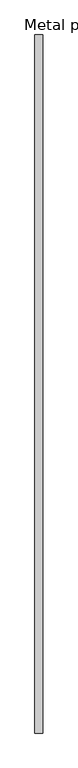
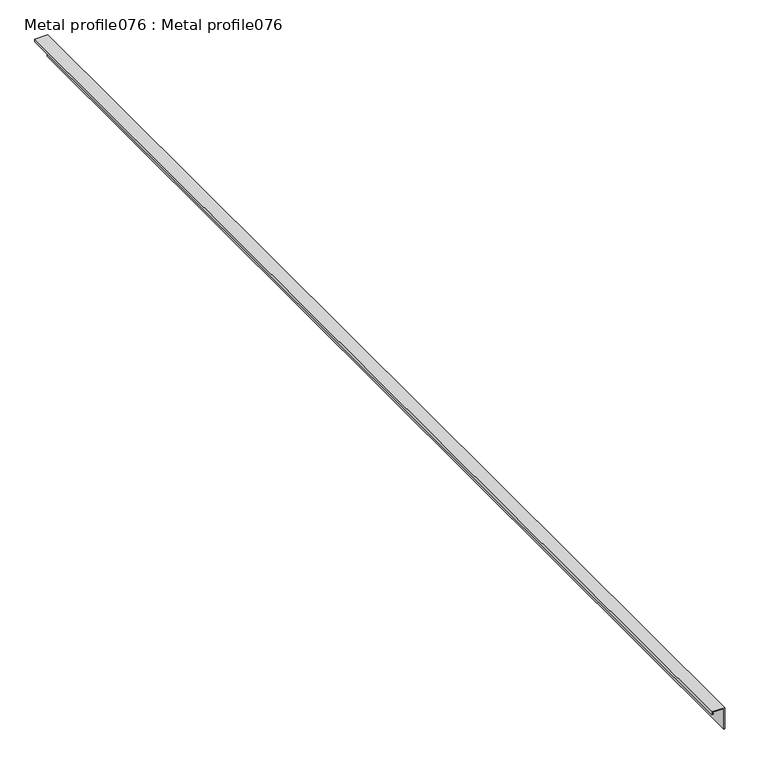
"""IFC4 building model written with IfcOpenShell, lengths in millimetres: proxy geometry, Metal profile076 : Metal profile076."""

from ifc_helpers import new_model, si_unit, frame, origin, place, context, project, spatial, polyline, outline, extrude, source, transform, mapped, element, save


def metal_profile076_metal_profile076_1ce1fb6e(model_context):
    return source(origin(), model_context, "Body", "SweptSolid", [
        extrude(outline(polyline([(40120.4288738, -9897.648077), (40083.5988738, -9897.648077), (40083.5988738, -9896.378077), (40121.6988738, -9896.378077), (40121.6988738, -9918.603077), (40116.9490738, -9918.603077), (40116.9490738, -9915.6006206), (40118.2190738, -9915.6006206), (40118.2190738, -9917.333077), (40120.4288738, -9917.333077), (40120.4288738, -9897.648077)])), frame((0.0, 7182.1531721, 0.0), z_axis=(0.0, 1.0, 0.0), x_axis=(0.0, 0.0, 1.0)), (0.0, 0.0, 1.0), 2000.0),
    ])


if __name__ == "__main__":
    model = new_model("IFC4")
    model_context = context("Model", 3, world=origin())
    ifc_project = project(units=[si_unit("LENGTHUNIT", "METRE", prefix="MILLI")], contexts=[model_context])
    site = spatial("IfcSite", under=ifc_project)
    building = spatial("IfcBuilding", under=site)
    placement = place(None, origin())
    metal_profile076_metal_profile076_shape = metal_profile076_metal_profile076_1ce1fb6e(model_context)
    element("IfcBuildingElementProxy", 1, Name="Metal profile076 : Metal profile076", ObjectType="Metal profile076 : Metal profile076", at=placement, inside=building, context=model_context, shape_type="MappedRepresentation", body=[
        mapped(metal_profile076_metal_profile076_shape, transform((0.0, 0.0, 0.0), x_axis=(1.0, 0.0, 0.0), y_axis=(0.0, 1.0, 0.0), z_axis=(0.0, 0.0, 1.0))),
    ])
    save(model, "model.ifc")

# Revit data of these elements
# Type "Metal profile076 : Metal profile076"
#   NameOverride = "Metal profile076"
# Element 1 (IfcBuildingElementProxy, "Metal profile076 : Metal profile076")
#   Materials on its faces: "COPPER STUCCO J BEAD"
# Materials
#   "COPPER STUCCO J BEAD": class "Unassigned", colour RGB 251 232 155, transparency 0, Cost = 0
